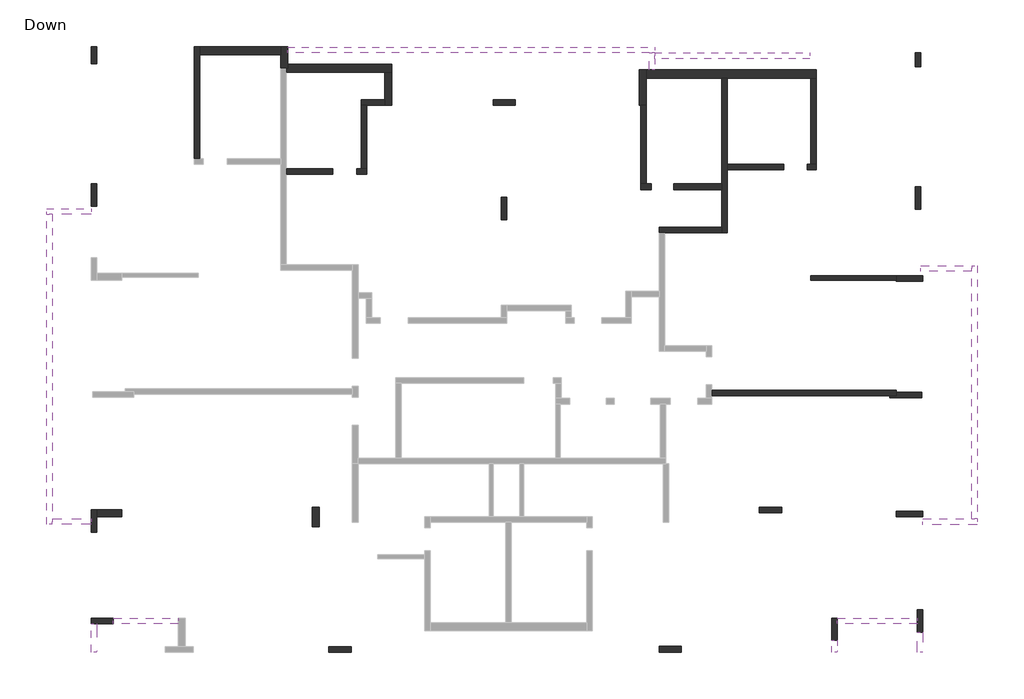
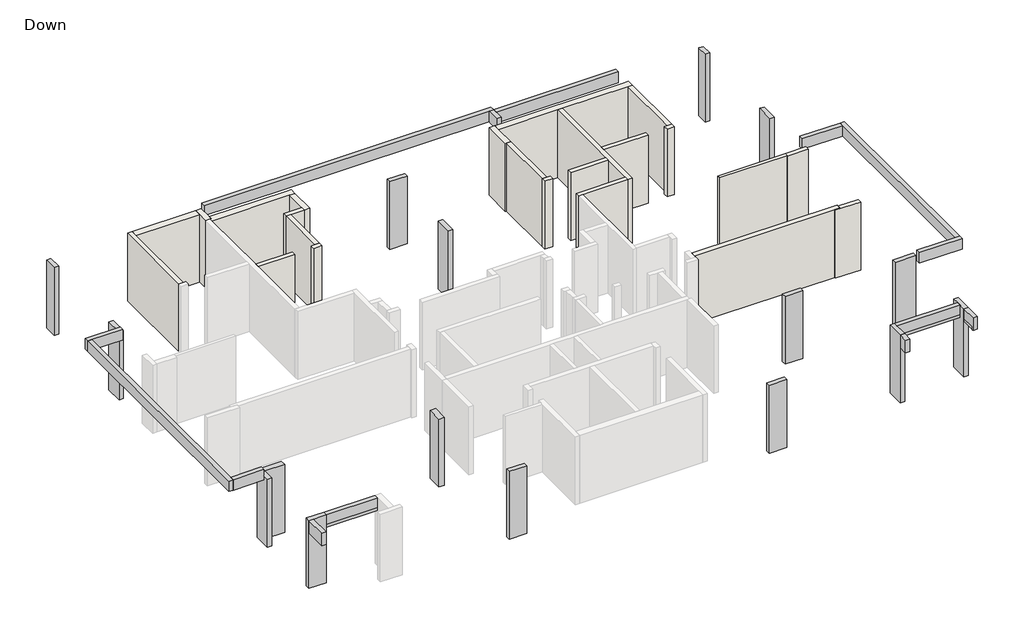
# One storey, part 2 of 2: 23 walls, 16 columns, 14 beams.
# Revit data of these elements (continued)
# Element 22 (IfcColumn, "Concrete Rectengular Column : 20/80") (continued)
#   Materials on its faces: "Concrete"
# Element 23 (IfcColumn, "Concrete Rectengular Column : 20/80")
#   Comments = ""
#   Mark = "C9"
#   SOFiSTiK_AMG_Comments = ""
#   SOFiSTiK_AMG_Scheduled = yes
#   SOFiSTiK_AMG_Adjusted = yes
#   Structural Material = Concrete
#   Phase Created = New Construction
#   Materials on its faces: "Concrete"
# Element 24 (IfcColumn, "Concrete Rectengular Column : 20/80")
#   Comments = ""
#   Mark = "C10"
#   SOFiSTiK_AMG_Comments = ""
#   SOFiSTiK_AMG_Scheduled = yes
#   SOFiSTiK_AMG_Adjusted = yes
#   Structural Material = Concrete
#   Phase Created = New Construction
#   Materials on its faces: "Concrete"
# Element 25 (IfcColumn, "Concrete Rectengular Column : 20/80")
#   Comments = ""
#   Mark = "C11"
#   SOFiSTiK_AMG_Comments = ""
#   SOFiSTiK_AMG_Scheduled = yes
#   SOFiSTiK_AMG_Adjusted = yes
#   Structural Material = Concrete
#   Phase Created = New Construction
#   Materials on its faces: "Concrete"
# Element 26 (IfcColumn, "Concrete Rectengular Column : 20/80")
#   Comments = ""
#   Mark = "C12"
#   SOFiSTiK_AMG_Comments = ""
#   SOFiSTiK_AMG_Scheduled = yes
#   SOFiSTiK_AMG_Adjusted = yes
#   Structural Material = Concrete
#   Phase Created = New Construction
#   Materials on its faces: "Concrete"
# Element 27 (IfcColumn, "Concrete Rectengular Column : 20/80")
#   Comments = ""
#   Mark = "C13"
#   SOFiSTiK_AMG_Comments = ""
#   SOFiSTiK_AMG_Scheduled = yes
#   SOFiSTiK_AMG_Adjusted = yes
#   Structural Material = Concrete
#   Phase Created = New Construction
#   Materials on its faces: "Concrete"
# Element 28 (IfcColumn, "Concrete Rectengular Column : 20/95")
#   Comments = ""
#   Mark = "C14"
#   SOFiSTiK_AMG_Comments = ""
#   SOFiSTiK_AMG_Scheduled = yes
#   SOFiSTiK_AMG_Adjusted = yes
#   Structural Material = Concrete
#   Phase Created = New Construction
#   Materials on its faces: "Concrete"
# Element 29 (IfcColumn, "Concrete Rectengular Column : 25/110")
#   Comments = ""
#   Mark = "C15"
#   SOFiSTiK_AMG_Comments = ""
#   SOFiSTiK_AMG_Scheduled = yes
#   SOFiSTiK_AMG_Adjusted = yes
#   Structural Material = Concrete
#   Phase Created = New Construction
#   Materials on its faces: "Concrete"
# Element 30 (IfcColumn, "Concrete Rectengular Column : 25/70")
#   Comments = ""
#   Mark = "C16"
#   SOFiSTiK_AMG_Comments = ""
#   SOFiSTiK_AMG_Scheduled = yes
#   SOFiSTiK_AMG_Adjusted = yes
#   Structural Material = Concrete
#   Phase Created = New Construction
#   Materials on its faces: "Concrete"
# Element 31 (IfcWall, "15")
#   Comments = ""
#   Mark = "W74"
#   SOFiSTiK_EdgeZones = "W76"
#   SOFiSTiK_AMG_Comments = ""
#   Top Offset = 0 cm
#   Base Offset = 0 cm
#   wall height = 327 cm
#   SOFiSTiK_AMG_Scheduled = yes
#   SOFiSTiK_AMG_Adjusted = yes
#   Phase Created = New Construction
#   Base Constraint = Down
#   Top Constraint = Typical Floor
#   Materials on its faces: "Concrete"
# Element 32 (IfcWall, "20")
#   Comments = ""
#   Mark = "W8"
#   SOFiSTiK_EdgeZones = "W9"
#   SOFiSTiK_AMG_Comments = ""
#   Top Offset = 0 cm
#   Base Offset = 0 cm
#   wall height = 327 cm
#   SOFiSTiK_AMG_Scheduled = yes
#   SOFiSTiK_AMG_Adjusted = yes
#   Phase Created = New Construction
#   Base Constraint = Down
#   Top Constraint = Typical Floor
#   Materials on its faces: "Concrete"
# Element 33 (IfcWall, "20")
#   Comments = ""
#   Mark = "W10"
#   SOFiSTiK_EdgeZones = "W11"
#   SOFiSTiK_AMG_Comments = ""
#   Top Offset = 0 cm
#   Base Offset = 0 cm
#   wall height = 327 cm
#   SOFiSTiK_AMG_Scheduled = yes
#   SOFiSTiK_AMG_Adjusted = yes
#   Phase Created = New Construction
#   Base Constraint = Down
#   Top Constraint = Typical Floor
#   Materials on its faces: "Concrete"
# Element 34 (IfcWall, "20")
#   Comments = ""
#   Mark = "W11"
#   SOFiSTiK_EdgeZones = "W12"
#   SOFiSTiK_AMG_Comments = ""
#   Top Offset = 0 cm
#   Base Offset = 0 cm
#   wall height = 327 cm
#   SOFiSTiK_AMG_Scheduled = yes
#   SOFiSTiK_AMG_Adjusted = yes
#   Phase Created = New Construction
#   Base Constraint = Down
#   Top Constraint = Typical Floor
#   Materials on its faces: "Concrete"
# Element 35 (IfcWall, "20")
#   Comments = ""
#   Mark = "W12"
#   SOFiSTiK_EdgeZones = "W13"
#   SOFiSTiK_AMG_Comments = ""
#   Top Offset = 0 cm
#   Base Offset = 0 cm
#   wall height = 327 cm
#   SOFiSTiK_AMG_Scheduled = yes
#   SOFiSTiK_AMG_Adjusted = yes
#   Phase Created = New Construction
#   Base Constraint = Down
#   Top Constraint = Typical Floor
#   Materials on its faces: "Concrete"
# Element 36 (IfcWall, "20")
#   Comments = ""
#   Mark = "W13"
#   SOFiSTiK_EdgeZones = "W14"
#   SOFiSTiK_AMG_Comments = ""
#   Top Offset = 0 cm
#   Base Offset = 0 cm
#   wall height = 327 cm
#   SOFiSTiK_AMG_Scheduled = yes
#   SOFiSTiK_AMG_Adjusted = yes
#   Phase Created = New Construction
#   Base Constraint = Down
#   Top Constraint = Typical Floor
#   Materials on its faces: "Concrete"
# Element 37 (IfcWall, "20")
#   Comments = ""
#   Mark = "W43"
#   SOFiSTiK_EdgeZones = "W45"
#   SOFiSTiK_AMG_Comments = ""
#   Top Offset = 0 cm
#   Base Offset = 0 cm
#   wall height = 327 cm
#   SOFiSTiK_AMG_Scheduled = yes
#   SOFiSTiK_AMG_Adjusted = yes
#   Phase Created = New Construction
#   Base Constraint = Down
#   Top Constraint = Typical Floor
#   Materials on its faces: "Concrete"
# Element 38 (IfcWall, "20")
#   Comments = ""
#   Mark = "W44"
#   SOFiSTiK_EdgeZones = "W46"
#   SOFiSTiK_AMG_Comments = ""
#   Top Offset = 0 cm
#   Base Offset = 0 cm
#   wall height = 327 cm
#   SOFiSTiK_AMG_Scheduled = yes
#   SOFiSTiK_AMG_Adjusted = yes
#   Phase Created = New Construction
#   Base Constraint = Down
#   Top Constraint = Typical Floor
#   Materials on its faces: "Concrete"
# Element 39 (IfcWall, "20")
#   Comments = ""
#   Mark = "W45"
#   SOFiSTiK_EdgeZones = "W47"
#   SOFiSTiK_AMG_Comments = ""
#   Top Offset = 0 cm
#   Base Offset = 0 cm
#   wall height = 327 cm
#   SOFiSTiK_AMG_Scheduled = yes
#   SOFiSTiK_AMG_Adjusted = yes
#   Phase Created = New Construction
#   Base Constraint = Down
#   Top Constraint = Typical Floor
#   Materials on its faces: "Concrete"
# Element 40 (IfcWall, "20")
#   Comments = ""
#   Mark = "W46"
#   SOFiSTiK_EdgeZones = "W48"
#   SOFiSTiK_AMG_Comments = ""
#   Top Offset = 0 cm
#   Base Offset = 0 cm
#   wall height = 327 cm
#   SOFiSTiK_AMG_Scheduled = yes
#   SOFiSTiK_AMG_Adjusted = yes
#   Phase Created = New Construction
#   Base Constraint = Down
#   Top Constraint = Typical Floor
#   Materials on its faces: "Concrete"
# Element 41 (IfcWall, "20")
#   Comments = ""
#   Mark = "W47"
#   SOFiSTiK_EdgeZones = "W49"
#   SOFiSTiK_AMG_Comments = ""
#   Top Offset = 0 cm
#   Base Offset = 0 cm
#   wall height = 327 cm
#   SOFiSTiK_AMG_Scheduled = yes
#   SOFiSTiK_AMG_Adjusted = yes
#   Phase Created = New Construction
#   Base Constraint = Down
#   Top Constraint = Typical Floor
#   Materials on its faces: "Concrete"
# Element 42 (IfcWall, "20")
#   Comments = ""
#   Mark = "W48"
#   SOFiSTiK_EdgeZones = "W50"
#   SOFiSTiK_AMG_Comments = ""
#   Top Offset = 0 cm
#   Base Offset = 0 cm
#   wall height = 327 cm
#   SOFiSTiK_AMG_Scheduled = yes
#   SOFiSTiK_AMG_Adjusted = yes
#   Phase Created = New Construction
#   Base Constraint = Down
#   Top Constraint = Typical Floor
#   Materials on its faces: "Concrete"
# Element 43 (IfcWall, "20")
#   Comments = ""
#   Mark = "W49"
#   SOFiSTiK_EdgeZones = "W51"
#   SOFiSTiK_AMG_Comments = ""
#   Top Offset = 0 cm
#   Base Offset = 0 cm
#   wall height = 327 cm
#   SOFiSTiK_AMG_Scheduled = yes
#   SOFiSTiK_AMG_Adjusted = yes
#   Phase Created = New Construction
#   Base Constraint = Down
#   Top Constraint = Typical Floor
#   Materials on its faces: "Concrete"
# Element 44 (IfcWall, "20")
#   Comments = ""
#   Mark = "W50"
#   SOFiSTiK_EdgeZones = "W52"
#   SOFiSTiK_AMG_Comments = ""
#   Top Offset = 0 cm
#   Base Offset = 0 cm
#   wall height = 327 cm
#   SOFiSTiK_AMG_Scheduled = yes
#   SOFiSTiK_AMG_Adjusted = yes
#   Phase Created = New Construction
#   Base Constraint = Down
#   Top Constraint = Typical Floor
#   Materials on its faces: "Concrete"
# Element 45 (IfcWall, "20")
#   Comments = ""
#   Mark = "W56"
#   SOFiSTiK_EdgeZones = "W58"
#   SOFiSTiK_AMG_Comments = ""
#   Top Offset = 0 cm
#   Base Offset = 0 cm
#   wall height = 327 cm
#   SOFiSTiK_AMG_Scheduled = yes
#   SOFiSTiK_AMG_Adjusted = yes
#   Phase Created = New Construction
#   Base Constraint = Down
#   Top Constraint = Typical Floor
#   Materials on its faces: "Concrete"
# Element 46 (IfcWall, "20")
#   Comments = ""
#   Mark = "W57"
#   SOFiSTiK_EdgeZones = "W59"
#   SOFiSTiK_AMG_Comments = ""
#   Top Offset = 0 cm
#   Base Offset = 0 cm
#   wall height = 327 cm
#   SOFiSTiK_AMG_Scheduled = yes
#   SOFiSTiK_AMG_Adjusted = yes
#   Phase Created = New Construction
#   Base Constraint = Down
#   Top Constraint = Typical Floor
#   Materials on its faces: "Concrete"
# Element 47 (IfcWall, "20")
#   Comments = ""
#   Mark = "W58"
#   SOFiSTiK_EdgeZones = "W60"
#   SOFiSTiK_AMG_Comments = ""
#   Top Offset = 0 cm
#   Base Offset = 0 cm
#   wall height = 327 cm
#   SOFiSTiK_AMG_Scheduled = yes
#   SOFiSTiK_AMG_Adjusted = yes
#   Phase Created = New Construction
#   Base Constraint = Down
#   Top Constraint = Typical Floor
#   Materials on its faces: "Concrete"
# Element 48 (IfcWall, "25")
#   Comments = ""
#   Mark = "W65"
#   SOFiSTiK_EdgeZones = "W67"
#   SOFiSTiK_AMG_Comments = ""
#   Top Offset = 0 cm
#   Base Offset = 0 cm
#   wall height = 327 cm
#   SOFiSTiK_AMG_Scheduled = yes
#   SOFiSTiK_AMG_Adjusted = yes
#   Phase Created = New Construction
#   Base Constraint = Down
#   Top Constraint = Typical Floor
#   Materials on its faces: "Concrete"
# Element 49 (IfcWall, "25")
#   Comments = ""
#   Mark = "W66"
#   SOFiSTiK_EdgeZones = "W68"
#   SOFiSTiK_AMG_Comments = ""
#   Top Offset = 0 cm
#   Base Offset = 0 cm
#   wall height = 327 cm
#   SOFiSTiK_AMG_Scheduled = yes
#   SOFiSTiK_AMG_Adjusted = yes
#   Phase Created = New Construction
#   Base Constraint = Down
#   Top Constraint = Typical Floor
#   Materials on its faces: "Concrete"
# Element 50 (IfcWall, "25")
#   Comments = ""
#   Mark = "W67"
#   SOFiSTiK_EdgeZones = "W69"
#   SOFiSTiK_AMG_Comments = ""
#   Top Offset = 0 cm
#   Base Offset = 0 cm
#   wall height = 327 cm
#   SOFiSTiK_AMG_Scheduled = yes
#   SOFiSTiK_AMG_Adjusted = yes
#   Phase Created = New Construction
#   Base Constraint = Down
#   Top Constraint = Typical Floor
#   Materials on its faces: "Concrete"
# Element 51 (IfcWall, "30")
#   Comments = ""
#   Mark = "W61"
#   SOFiSTiK_EdgeZones = "W63"
#   SOFiSTiK_AMG_Comments = ""
#   Top Offset = 0 cm
#   Base Offset = 0 cm
#   wall height = 327 cm
#   SOFiSTiK_AMG_Scheduled = yes
#   SOFiSTiK_AMG_Adjusted = yes
#   Phase Created = New Construction
#   Base Constraint = Down
#   Top Constraint = Typical Floor
#   Materials on its faces: "Concrete"
# Element 52 (IfcWall, "30")
#   Comments = ""
#   Mark = "W62"
#   SOFiSTiK_EdgeZones = "W64"
#   SOFiSTiK_AMG_Comments = ""
#   Top Offset = 0 cm
#   Base Offset = 0 cm
#   wall height = 327 cm
#   SOFiSTiK_AMG_Scheduled = yes
#   SOFiSTiK_AMG_Adjusted = yes
#   Phase Created = New Construction
#   Base Constraint = Down
#   Top Constraint = Typical Floor
#   Materials on its faces: "Concrete"
# Element 53 (IfcWall, "30")
#   Comments = ""
#   Mark = "W64"
#   SOFiSTiK_EdgeZones = "W66"
#   SOFiSTiK_AMG_Comments = ""
#   Top Offset = 0 cm
#   Base Offset = 0 cm
#   wall height = 327 cm
#   SOFiSTiK_AMG_Scheduled = yes
#   SOFiSTiK_AMG_Adjusted = yes
#   Phase Created = New Construction
#   Base Constraint = Down
#   Top Constraint = Typical Floor
#   Materials on its faces: "Concrete"
# Materials
#   "Concrete": class "Concrete", colour RGB 192 192 192, transparency 0, Keynote = "01000", Description = "Cast-in-place concrete", Cost = 0
